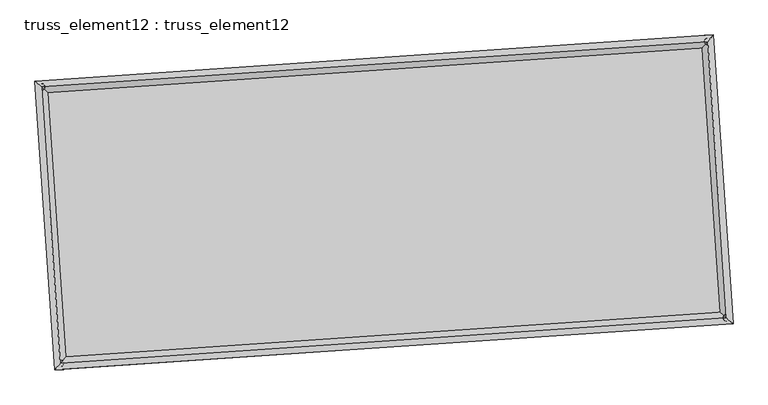
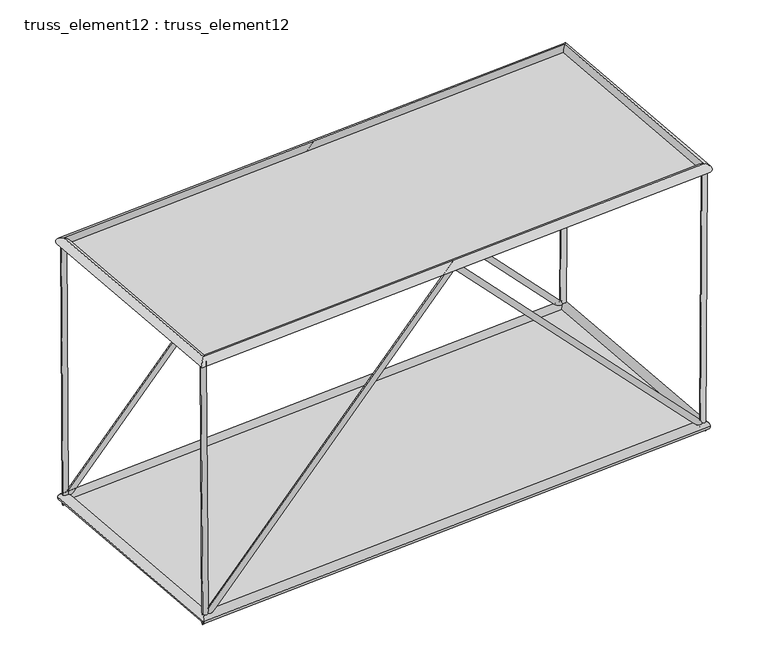
"""IFC4 building model written with IfcOpenShell, lengths in millimetres: plate geometry, truss_element12 : truss_element12."""

import ifcopenshell
import ifcopenshell.guid

model = None  # the IFC model being written
_history = None  # IfcOwnerHistory: only IFC2X3 demands one
_inside = {}  # id of a spatial element -> (the spatial element, [elements in it])
_under = {}  # id of a project, library or spatial element -> (it, [spatial elements below it])
_declared = {}  # id of a project -> (the project, [libraries it declares])
_typed = {}  # id of a type object -> (the type object, [elements of that type])
_made_of = {}  # id of a material, layer set ... -> (it, [elements and type objects made of it])


def new_model(schema):
    """Start an empty IFC model of exactly this schema.

    Asked for "IFC4X3", IfcOpenShell would pick the latest addendum, in which some entities
    have other attributes; the version numbers below select the first issue.
    IFC2X3 requires an IfcOwnerHistory on every rooted entity: one is made here for all.
    """
    global model, _history
    if schema == "IFC4X3":
        model = ifcopenshell.file(schema_version=(4, 3, 0, 0))
    else:
        model = ifcopenshell.file(schema=schema)
    _inside.clear()
    _under.clear()
    _declared.clear()
    _typed.clear()
    _made_of.clear()
    _history = None
    if model.schema == "IFC2X3":
        org = make("IfcOrganization", Name="unknown")
        user = make(
            "IfcPersonAndOrganization",
            ThePerson=make("IfcPerson", FamilyName="unknown"),
            TheOrganization=org,
        )
        app = make(
            "IfcApplication",
            ApplicationDeveloper=org,
            Version="unknown",
            ApplicationFullName="unknown",
            ApplicationIdentifier="unknown",
        )
        _history = make(
            "IfcOwnerHistory",
            OwningUser=user,
            OwningApplication=app,
            ChangeAction="ADDED",
            CreationDate=0,
        )
    return model


def make(cls, **values):
    """One entity of the class cls with the attributes given. An attribute that is None is left unset."""
    return model.create_entity(
        cls, **{name: value for name, value in values.items() if value is not None}
    )


def rooted(cls, **values):
    """An entity with a GlobalId (a new one), such as an element, a storey or a relation."""
    return make(cls, GlobalId=ifcopenshell.guid.new(), OwnerHistory=_history, **values)


def si_unit(unit_type, name, prefix=None):
    """IfcSIUnit, for example si_unit("LENGTHUNIT", "METRE", prefix="MILLI")."""
    return make("IfcSIUnit", UnitType=unit_type, Prefix=prefix, Name=name)


def assignment(units):
    """IfcUnitAssignment: the units of a project."""
    return None if units is None else make("IfcUnitAssignment", Units=units)


def point(xyz):
    """IfcCartesianPoint."""
    return None if xyz is None else make("IfcCartesianPoint", Coordinates=xyz)


def direction(xyz):
    """IfcDirection."""
    return None if xyz is None else make("IfcDirection", DirectionRatios=xyz)


def frame(location, z_axis=None, x_axis=None):
    """IfcAxis2Placement3D, a coordinate frame: its origin and axes. An axis left out is left unset."""
    return make(
        "IfcAxis2Placement3D",
        Location=point(location),
        Axis=direction(z_axis),
        RefDirection=direction(x_axis),
    )


def origin():
    """The frame at (0, 0, 0) with its axes left unset."""
    return frame((0.0, 0.0, 0.0))


def origin_with_axes():
    """The frame at (0, 0, 0) with the z axis (0, 0, 1) and the x axis (1, 0, 0) written out."""
    return frame((0.0, 0.0, 0.0), z_axis=(0.0, 0.0, 1.0), x_axis=(1.0, 0.0, 0.0))


def place(relative_to, where):
    """IfcLocalPlacement: puts the frame where relative to a parent placement (None: the world)."""
    return make(
        "IfcLocalPlacement", PlacementRelTo=relative_to, RelativePlacement=where
    )


def context(
    kind, dimensions, precision=None, world=None, true_north=None, identifier=None
):
    """IfcGeometricRepresentationContext, for example the 3D "Model" context."""
    return make(
        "IfcGeometricRepresentationContext",
        ContextIdentifier=identifier,
        ContextType=kind,
        CoordinateSpaceDimension=dimensions,
        Precision=precision,
        WorldCoordinateSystem=world,
        TrueNorth=true_north,
    )


def project(units=None, contexts=None):
    """IfcProject with its units and contexts."""
    return rooted(
        "IfcProject",
        Name="project",
        RepresentationContexts=contexts,
        UnitsInContext=assignment(units),
    )


def spatial(cls, under=None, at=None, **own):
    """A site, building, storey or space (cls), placed at a placement, below another one or the project."""
    s = rooted(cls, ObjectPlacement=at, **own)
    if under is not None:
        _under.setdefault(under.id(), (under, []))[1].append(s)
    return s


def polyline(points):
    """IfcPolyline through the points."""
    return make("IfcPolyline", Points=[point(p) for p in points])


def circle_curve(where, radius):
    """IfcCircle in the frame where."""
    return make("IfcCircle", Position=where, Radius=radius)


def ellipse_curve(where, semi_axis1, semi_axis2):
    """IfcEllipse in the frame where."""
    return make(
        "IfcEllipse", Position=where, SemiAxis1=semi_axis1, SemiAxis2=semi_axis2
    )


def outline(outer, holes=None, kind="AREA"):
    """IfcArbitraryClosedProfileDef: a profile drawn as a closed curve; with holes, ...WithVoids."""
    if holes is None:
        return make("IfcArbitraryClosedProfileDef", ProfileType=kind, OuterCurve=outer)
    return make(
        "IfcArbitraryProfileDefWithVoids",
        ProfileType=kind,
        OuterCurve=outer,
        InnerCurves=holes,
    )


def extrude(swept, where, along, depth):
    """IfcExtrudedAreaSolid: the profile swept, set in the frame where, extruded along a direction by depth."""
    return make(
        "IfcExtrudedAreaSolid",
        SweptArea=swept,
        Position=where,
        ExtrudedDirection=direction(along),
        Depth=depth,
    )


def shape(context_of_items, identifier, shape_type, items):
    """IfcShapeRepresentation: the items that make up one representation, for example the "Body"."""
    return make(
        "IfcShapeRepresentation",
        ContextOfItems=context_of_items,
        RepresentationIdentifier=identifier,
        RepresentationType=shape_type,
        Items=items,
    )


def source(mapping_origin, context_of_items, identifier, shape_type, items):
    """IfcRepresentationMap: a shape defined once, which mapped items show again and again."""
    return make(
        "IfcRepresentationMap",
        MappingOrigin=mapping_origin,
        MappedRepresentation=shape(context_of_items, identifier, shape_type, items),
    )


def transform(
    local_origin,
    x_axis=None,
    y_axis=None,
    z_axis=None,
    scale=None,
    scale2=None,
    scale3=None,
    uniform=True,
):
    """IfcCartesianTransformationOperator3D, or its non-uniform kind. x_axis, y_axis, z_axis: its Axis1, 2, 3."""
    if uniform:
        return make(
            "IfcCartesianTransformationOperator3D",
            Axis1=direction(x_axis),
            Axis2=direction(y_axis),
            LocalOrigin=point(local_origin),
            Scale=scale,
            Axis3=direction(z_axis),
        )
    return make(
        "IfcCartesianTransformationOperator3DnonUniform",
        Axis1=direction(x_axis),
        Axis2=direction(y_axis),
        LocalOrigin=point(local_origin),
        Scale=scale,
        Axis3=direction(z_axis),
        Scale2=scale2,
        Scale3=scale3,
    )


def mapped(mapping_source, mapping_target):
    """IfcMappedItem: shows the shape of a source again, moved by a transform."""
    return make(
        "IfcMappedItem", MappingSource=mapping_source, MappingTarget=mapping_target
    )


def made_of(thing, what):
    """Note that an element or type object is made of a material, layer set ...; save() writes the relation."""
    if what is not None:
        _made_of.setdefault(what.id(), (what, []))[1].append(thing)
    return thing


def element(
    cls,
    number,
    at=None,
    inside=None,
    cuts=None,
    type_object=None,
    material=None,
    context=None,
    identifier="Body",
    shape_type=None,
    held_by="IfcProductDefinitionShape",
    body=None,
    shapes=None,
    **own,
):
    """One element of the class cls, such as IfcWall. Its Tag is "e" and its number.

    at: its placement. inside: the storey or other place that contains it. cuts: it is an
    opening in that element (IfcRelVoidsElement). A single representation is given by context,
    identifier, shape_type and body (its items); several are given by shapes. held_by: the class
    of the entity that holds the representations. save() writes the other relations.
    """
    e = rooted(cls, Tag="e%d" % number, ObjectPlacement=at, **own)
    if body is not None:
        shapes = [shape(context, identifier, shape_type, body)]
    if shapes is not None:
        e.Representation = make(held_by, Representations=shapes)
    if inside is not None:
        _inside.setdefault(inside.id(), (inside, []))[1].append(e)
    if cuts is not None:
        rooted(
            "IfcRelVoidsElement", RelatingBuildingElement=cuts, RelatedOpeningElement=e
        )
    if type_object is not None:
        _typed.setdefault(type_object.id(), (type_object, []))[1].append(e)
    return made_of(e, material)


def aggregate(whole, parts):
    """IfcRelAggregates: a whole, such as a stair, and the parts it consists of."""
    return rooted("IfcRelAggregates", RelatingObject=whole, RelatedObjects=parts)


def save(model, path):
    """Write the relations noted so far, then the file.

    IfcRelAggregates (storeys below a building ...), IfcRelContainedInSpatialStructure (elements
    in a storey), IfcRelDefinesByType, IfcRelAssociatesMaterial and IfcRelDeclares: one each for
    every whole, place, type object, material and project.
    """
    for whole, parts in _under.values():
        aggregate(whole, parts)
    for where, things in _inside.values():
        rooted(
            "IfcRelContainedInSpatialStructure",
            RelatedElements=things,
            RelatingStructure=where,
        )
    for kind, things in _typed.values():
        rooted("IfcRelDefinesByType", RelatedObjects=things, RelatingType=kind)
    for what, things in _made_of.values():
        rooted("IfcRelAssociatesMaterial", RelatedObjects=things, RelatingMaterial=what)
    for by, libraries in _declared.values():
        rooted("IfcRelDeclares", RelatingContext=by, RelatedDefinitions=libraries)
    model.write(path)


def plane_surface(at):
    """IfcPlane: the flat surface through the origin of the frame at, square to its z axis."""
    return make("IfcPlane", Position=at)


def cylinder_surface(at, radius):
    """IfcCylindricalSurface: all points at the distance radius from the z axis of the frame at."""
    return make("IfcCylindricalSurface", Position=at, Radius=radius)


def advanced_brep(points, edges, surfaces, faces):
    """IfcAdvancedBrep: a solid bounded by faces that lie on surfaces and meet in shared edges.

    An edge is (start, end): straight between two places in points (the first is 0);
    or (start, end, curve); or (start, end, curve, False) where it runs against its curve.
    A face is (place in surfaces, loops), or (place, loops, False) where it looks against
    its surface's normal. A loop lists edges by number (the first is 1), with a minus sign
    where the edge is run from its end to its start. The first loop is the outer one.
    """
    corners = [point(p) for p in points]
    vertices = [make("IfcVertexPoint", VertexGeometry=c) for c in corners]
    made = []
    for start, end, *more in edges:
        made.append(
            make(
                "IfcEdgeCurve",
                EdgeStart=vertices[start],
                EdgeEnd=vertices[end],
                EdgeGeometry=more[0] if more else make("IfcPolyline", Points=[corners[start], corners[end]]),
                SameSense=more[1] if len(more) > 1 else True,
            )
        )
    hull = []
    for where, loops, *sense in faces:
        bounds = []
        for j, loop in enumerate(loops):
            ring = [make("IfcOrientedEdge", EdgeElement=made[abs(k) - 1], Orientation=k > 0) for k in loop]
            bounds.append(
                make(
                    "IfcFaceOuterBound" if j == 0 else "IfcFaceBound",
                    Bound=make("IfcEdgeLoop", EdgeList=ring),
                    Orientation=True,
                )
            )
        hull.append(make("IfcAdvancedFace", Bounds=bounds, FaceSurface=surfaces[where], SameSense=sense[0] if sense else True))
    return make("IfcAdvancedBrep", Outer=make("IfcClosedShell", CfsFaces=hull))


def truss_element12_truss_element12_7878418a(model_context):
    return source(origin(), model_context, "Body", "SolidModel", [
        advanced_brep(
        [(-3697.7330559, 2273.9880634, 5000.2199286), (-3796.8342671, 2260.6269358, 4999.5640296), (-3665.7497354, 2276.1688844, 123.3649597), (-3763.2371475, 2262.9177957, -123.3649597), (1063.4710215, 2598.6364704, 5072.016746), (1063.9229343, 2592.0634919, 4927.7704366), (5793.1764667, 2921.1371054, 123.3684641), (5891.5845103, 2921.2433831, -123.3684641), (5824.6787759, 2923.2851281, 5000.2182213), (5924.6764587, 2923.4997973, 4999.5721856)],
        [
            (0, 1, circle_curve(frame((-3747.2836615, 2267.3074996, 4999.8919791), z_axis=(-0.0065580440171227215, -0.0004471680920716447, 0.9999783958163132), x_axis=(-0.13361132201156306, 0.9910337164155191, -0.0004330796311214912)), 50.0)),
            (1, 0, circle_curve(frame((-3747.2836615, 2267.3074996, 4999.8919791), z_axis=(-0.0065580440171227215, -0.0004471680920716447, 0.9999783958163132), x_axis=(-0.13361132201156306, 0.9910337164155191, -0.0004330796311214912)), 50.0)),
            (0, 2),
            (2, 3, ellipse_curve(frame((-3714.4934414, 2269.54334, 0.0), z_axis=(-0.9270094873495339, -0.06320925304940259, 0.36967282925972605), x_axis=(0.36881644373245154, 0.025148191295556746, 0.9291619876572165)), 133.0592395, 50.0)),
            (3, 1),
            (3, 2, ellipse_curve(frame((-3714.4934414, 2269.54334, 0.0), z_axis=(-0.9270094873495339, -0.06320925304940259, 0.36967282925972605), x_axis=(0.36881644373245154, 0.025148191295556746, 0.9291619876572165)), 133.0592395, 50.0)),
            (2, 4),
            (4, 5, ellipse_curve(frame((1063.6969779, 2595.3499811, 4999.8935913), z_axis=(-0.9976833957434984, -0.06802823820610858, -2.5773915168840048e-05), x_axis=(2.571420721554706e-05, 1.7533540442212808e-06, -0.9999999996678525)), 72.2802032, 50.0)),
            (5, 3),
            (5, 4, ellipse_curve(frame((1063.6969779, 2595.3499811, 4999.8935913), z_axis=(-0.9976833957434984, -0.06802823820610858, -2.5773915168840048e-05), x_axis=(2.571420721554706e-05, 1.7533540442212808e-06, -0.9999999996678525)), 72.2802032, 50.0)),
            (4, 6),
            (6, 7, ellipse_curve(frame((5842.3804885, 2921.1902443, 0.0), z_axis=(-0.9269817502517963, -0.06320736176214367, -0.3697426998862667), x_axis=(-0.36888615249642426, -0.025152944471190097, 0.929134186154408)), 133.0670008, 50.0)),
            (7, 5),
            (7, 6, ellipse_curve(frame((5842.3804885, 2921.1902443, 0.0), z_axis=(-0.9269817502517963, -0.06320736176214367, -0.3697426998862667), x_axis=(-0.36888615249642426, -0.025152944471190097, 0.929134186154408)), 133.0670008, 50.0)),
            (8, 9, circle_curve(frame((5874.6776173, 2923.3924627, 4999.8952035), z_axis=(0.0064594257599789005, 0.0004404436879936221, 0.9999790406944584), x_axis=(-0.002149492172002672, 0.9999975988590792, -0.00042656708586943926)), 50.0)),
            (9, 8, circle_curve(frame((5874.6776173, 2923.3924627, 4999.8952035), z_axis=(0.0064594257599789005, 0.0004404436879936221, 0.9999790406944584), x_axis=(-0.002149492172002672, 0.9999975988590792, -0.00042656708586943926)), 50.0)),
            (6, 8),
            (9, 7),
        ],
        [
            plane_surface(frame((-3747.2836615, 2317.3074946, 4999.914338), z_axis=(-0.006558044017122149, -0.0004471680920756006, 0.9999783958163133), x_axis=(0.9999784957981195, -2.932611094408344e-06, 0.0065580433614229605))),
            cylinder_surface(frame((-3747.2836615, 2267.3074996, 4999.8919791), z_axis=(-0.0065580440171227215, -0.0004471680920716447, 0.9999783958163132), x_axis=(-0.13361132201156306, 0.9910337164155191, -0.0004330796311214912)), 50.0),
            cylinder_surface(frame((-3714.4934414, 2269.54334, 0.0), z_axis=(-0.6901312584427534, -0.047057427078693426, -0.722152646382297), x_axis=(-0.02041166390988012, 0.9987523707892875, -0.045574837566446924)), 50.0),
            cylinder_surface(frame((1063.6969779, 2595.3499811, 4999.8935913), z_axis=(-0.6901683966914209, -0.047059959394698786, 0.7221169880498334), x_axis=(-0.11534684875831876, 0.9922791014168952, -0.04557729009939607)), 50.0),
            plane_surface(frame((5874.6776173, 2873.3924675, 4999.9172261), z_axis=(0.006459425759978055, 0.0004404436879920798, 0.9999790406944582), x_axis=(0.9999791376918077, -2.845072659241059e-06, -0.006459425133417806))),
            cylinder_surface(frame((5842.3804885, 2921.1902443, 0.0), z_axis=(-0.0064594257599789005, -0.0004404436879936221, -0.9999790406944584), x_axis=(-0.002149492172002672, 0.9999975988590792, -0.00042656708586943926)), 50.0),
        ],
        [
            (0, [[1, 2]]),
            (1, [[-1, 3, 4, 5]]),
            (1, [[-2, -5, 6, -3]]),
            (2, [[-4, 7, 8, 9]]),
            (2, [[-6, -9, 10, -7]]),
            (3, [[-8, 11, 12, 13]]),
            (3, [[-10, -13, 14, -11]]),
            (4, [[15, 16]]),
            (5, [[-12, 17, -16, 18]]),
            (5, [[-14, -18, -15, -17]]),
        ],
    ),
        advanced_brep(
        [(-3425.620103, -1716.7455209, 5000.2199286), (-3524.7213142, -1730.1066485, 4999.5640296), (-3393.6367824, -1714.5646999, 123.3649597), (-3491.1241946, -1727.8157886, -123.3649597), (1335.5839744, -1392.0971139, 5072.016746), (1336.0358872, -1398.6700924, 4927.7704366), (6065.2894196, -1069.5964789, 123.3684641), (6163.6974632, -1069.4902012, -123.3684641), (6096.7917288, -1067.4484562, 5000.2182213), (6196.7894116, -1067.233787, 4999.5721856)],
        [
            (0, 1, circle_curve(frame((-3475.1707086, -1723.4260847, 4999.8919791), z_axis=(-0.006558044017122952, -0.00044716809207167603, 0.9999783958163132), x_axis=(-0.1336113220115621, 0.9910337164155192, -0.0004330796311214846)), 50.0)),
            (1, 0, circle_curve(frame((-3475.1707086, -1723.4260847, 4999.8919791), z_axis=(-0.006558044017122952, -0.00044716809207167603, 0.9999783958163132), x_axis=(-0.1336113220115621, 0.9910337164155192, -0.0004330796311214846)), 50.0)),
            (0, 2),
            (2, 3, ellipse_curve(frame((-3442.3804885, -1721.1902443, 0.0), z_axis=(-0.927009487349534, -0.06320925304940223, 0.3696728292597261), x_axis=(0.3688164437324516, 0.025148191295556586, 0.9291619876572165)), 133.0592395, 50.0)),
            (3, 1),
            (3, 2, ellipse_curve(frame((-3442.3804885, -1721.1902443, 0.0), z_axis=(-0.927009487349534, -0.06320925304940223, 0.3696728292597261), x_axis=(0.3688164437324516, 0.025148191295556586, 0.9291619876572165)), 133.0592395, 50.0)),
            (2, 4),
            (4, 5, ellipse_curve(frame((1335.8099308, -1395.3836032, 4999.8935913), z_axis=(-0.9976833957434985, -0.06802823820610843, -2.5773915170605434e-05), x_axis=(2.5714207217238277e-05, 1.7533540445864214e-06, -0.9999999996678526)), 72.2802032, 50.0)),
            (5, 3),
            (5, 4, ellipse_curve(frame((1335.8099308, -1395.3836032, 4999.8935913), z_axis=(-0.9976833957434985, -0.06802823820610843, -2.5773915170605434e-05), x_axis=(2.5714207217238277e-05, 1.7533540445864214e-06, -0.9999999996678526)), 72.2802032, 50.0)),
            (4, 6),
            (6, 7, ellipse_curve(frame((6114.4934414, -1069.54334, 0.0), z_axis=(-0.9269817502517956, -0.06320736176214367, -0.3697426998862684), x_axis=(-0.3688861524964258, -0.025152944471190226, 0.9291341861544073)), 133.0670008, 50.0)),
            (7, 5),
            (7, 6, ellipse_curve(frame((6114.4934414, -1069.54334, 0.0), z_axis=(-0.9269817502517956, -0.06320736176214367, -0.3697426998862684), x_axis=(-0.3688861524964258, -0.025152944471190226, 0.9291341861544073)), 133.0670008, 50.0)),
            (8, 9, circle_curve(frame((6146.7905702, -1067.3411216, 4999.8952035), z_axis=(0.006459425759979071, 0.0004404436879936256, 0.9999790406944583), x_axis=(-0.002149492172003178, 0.9999975988590791, -0.00042656708586943915)), 50.0)),
            (9, 8, circle_curve(frame((6146.7905702, -1067.3411216, 4999.8952035), z_axis=(0.006459425759979071, 0.0004404436879936256, 0.9999790406944583), x_axis=(-0.002149492172003178, 0.9999975988590791, -0.00042656708586943915)), 50.0)),
            (6, 8),
            (9, 7),
        ],
        [
            plane_surface(frame((-3475.1707086, -1673.4260897, 4999.914338), z_axis=(-0.006558044017122149, -0.00044716809207560177, 0.9999783958163133), x_axis=(0.9999784957981195, -2.932611094408344e-06, 0.0065580433614229605))),
            cylinder_surface(frame((-3475.1707086, -1723.4260847, 4999.8919791), z_axis=(-0.0065580440171229505, -0.0004471680920716759, 0.999978395816313), x_axis=(-0.1336113220115621, 0.9910337164155192, -0.0004330796311214846)), 50.0),
            cylinder_surface(frame((-3442.3804885, -1721.1902443, 0.0), z_axis=(-0.6901312584427537, -0.04705742707869316, -0.7221526463822968), x_axis=(-0.020411663909880064, 0.9987523707892874, -0.045574837566446605)), 50.0),
            cylinder_surface(frame((1335.8099308, -1395.3836032, 4999.8935913), z_axis=(-0.6901683966914235, -0.047059959394698994, 0.7221169880498306), x_axis=(-0.1153468487583182, 0.9922791014168953, -0.045577290099395824)), 50.0),
            plane_surface(frame((6146.7905702, -1117.3411168, 4999.9172261), z_axis=(0.006459425759978055, 0.00044044368799207986, 0.9999790406944582), x_axis=(0.9999791376918077, -2.8450726587969697e-06, -0.006459425133417806))),
            cylinder_surface(frame((6114.4934414, -1069.54334, 0.0), z_axis=(-0.006459425759979071, -0.0004404436879936256, -0.9999790406944583), x_axis=(-0.002149492172003178, 0.9999975988590791, -0.00042656708586943915)), 50.0),
        ],
        [
            (0, [[1, 2]]),
            (1, [[-1, 3, 4, 5]]),
            (1, [[-2, -5, 6, -3]]),
            (2, [[-4, 7, 8, 9]]),
            (2, [[-6, -9, 10, -7]]),
            (3, [[-8, 11, 12, 13]]),
            (3, [[-10, -13, 14, -11]]),
            (4, [[15, 16]]),
            (5, [[-12, 17, -16, 18]]),
            (5, [[-14, -18, -15, -17]]),
        ],
    ),
        advanced_brep(
        [(-3475.1698571, -1723.425141, 4909.8919791), (-3475.1715601, -1723.4270284, 5089.8919791), (-3747.2846332, 2267.308319, 5089.8919791), (-3747.2826898, 2267.3066802, 4909.8919791), (5874.6784087, 2923.3934023, 5089.8952035), (5874.6768259, 2923.3915231, 4909.8952035), (6146.7914819, -1067.3419451, 5089.8952035), (6146.7896586, -1067.3402981, 4909.8952035)],
        [
            (0, 1, ellipse_curve(frame((-3475.1707086, -1723.4260847, 4999.8919791), z_axis=(-0.7535719234054182, 0.6573654662780838, -2.364078017319096e-07), x_axis=(-0.6573654662780416, -0.7535719234054551, -2.3640780134907803e-07)), 127.2792206, 90.0)),
            (1, 2),
            (2, 3, ellipse_curve(frame((-3747.2836615, 2267.3074996, 4999.8919791), z_axis=(-0.6573654662780415, -0.7535719234054551, -2.3640779880847992e-07), x_axis=(0.7535719234054182, -0.6573654662780839, 2.3640779919131162e-07)), 127.2792206, 90.0)),
            (3, 0),
            (1, 0, ellipse_curve(frame((-3475.1707086, -1723.4260847, 4999.8919791), z_axis=(-0.7535719234054182, 0.6573654662780838, -2.364078017319096e-07), x_axis=(-0.6573654662780416, -0.7535719234054551, -2.3640780134907803e-07)), 127.2792206, 90.0)),
            (3, 2, ellipse_curve(frame((-3747.2836615, 2267.3074996, 4999.8919791), z_axis=(-0.6573654662780415, -0.7535719234054551, -2.3640779880847992e-07), x_axis=(0.7535719234054182, -0.6573654662780839, 2.3640779919131162e-07)), 127.2792206, 90.0)),
            (2, 4),
            (4, 5, ellipse_curve(frame((5874.6776173, 2923.3924627, 4999.8952035), z_axis=(-0.753571923405421, 0.6573654662780805, -2.364078053169509e-07), x_axis=(-0.6573654662780386, -0.7535719234054576, -2.3640779268284074e-07)), 127.2792206, 90.0)),
            (5, 3),
            (5, 4, ellipse_curve(frame((5874.6776173, 2923.3924627, 4999.8952035), z_axis=(-0.753571923405421, 0.6573654662780805, -2.364078053169509e-07), x_axis=(-0.6573654662780386, -0.7535719234054576, -2.3640779268284074e-07)), 127.2792206, 90.0)),
            (4, 6),
            (6, 7, ellipse_curve(frame((6146.7905702, -1067.3411216, 4999.8952035), z_axis=(0.6573654662780387, 0.7535719234054576, 2.3640779522343875e-07), x_axis=(-0.7535719234054211, 0.6573654662780807, -2.364078078575489e-07)), 127.2792206, 90.0)),
            (7, 5),
            (7, 6, ellipse_curve(frame((6146.7905702, -1067.3411216, 4999.8952035), z_axis=(0.6573654662780387, 0.7535719234054576, 2.3640779522343875e-07), x_axis=(-0.7535719234054211, 0.6573654662780807, -2.364078078575489e-07)), 127.2792206, 90.0)),
            (6, 1),
            (0, 7),
        ],
        [
            cylinder_surface(frame((-3475.1707086, -1723.4260847, 4999.8919791), z_axis=(0.06802823822870056, -0.9976833960748767, 0.0), x_axis=(-0.9976833960234631, -0.06802823822519488, -1.0152132427543063e-05)), 90.0),
            cylinder_surface(frame((-3747.2836615, 2267.3074996, 4999.8919791), z_axis=(-0.9976833960748208, -0.06802823822869773, -3.3433111559642525e-07), x_axis=(-0.06802823822214815, 0.9976833960270169, -9.817801312233482e-06)), 90.0),
            cylinder_surface(frame((5874.6776173, 2923.3924627, 4999.8952035), z_axis=(-0.06802823822870865, 0.9976833960748761, 0.0), x_axis=(0.9976833960300122, 0.06802823822564956, -9.48347018771953e-06)), 90.0),
            cylinder_surface(frame((6146.7905702, -1067.3411216, 4999.8952035), z_axis=(0.997683396074821, 0.06802823822869727, 3.3433111918937347e-07), x_axis=(0.06802823822869727, -0.9976833960265705, -9.81780129795915e-06)), 90.0),
        ],
        [
            (0, [[1, 2, 3, 4]]),
            (0, [[5, -4, 6, -2]]),
            (1, [[-3, 7, 8, 9]]),
            (1, [[-6, -9, 10, -7]]),
            (2, [[-8, 11, 12, 13]]),
            (2, [[-10, -13, 14, -11]]),
            (3, [[-12, 15, -1, 16]]),
            (3, [[-14, -16, -5, -15]]),
        ],
    ),
        advanced_brep(
        [(-3358.7115243, -1625.2761972, 0.0), (-3526.0494527, -1817.1042913, 0.0), (-3810.4074885, 2353.2123043, 0.0), (-3618.5793943, 2185.8743758, 0.0), (5926.0494527, 3017.1042913, 0.0), (5758.7115243, 2825.2761972, 0.0), (6210.4074885, -1153.2123043, 0.0), (6018.5793943, -985.8743758, 0.0)],
        [
            (0, 1, ellipse_curve(frame((-3442.3804885, -1721.1902443, 0.0), z_axis=(-0.7535719234054593, 0.6573654662780792, 0.0), x_axis=(-0.6573654662780792, -0.7535719234054593, 0.0)), 127.2792206, 90.0)),
            (1, 2),
            (2, 3, ellipse_curve(frame((-3714.4934414, 2269.54334, 0.0), z_axis=(-0.6573654662780791, -0.7535719234054593, 0.0), x_axis=(0.7535719234054593, -0.6573654662780793, 0.0)), 127.2792206, 90.0)),
            (3, 0),
            (1, 0, ellipse_curve(frame((-3442.3804885, -1721.1902443, 0.0), z_axis=(-0.7535719234054593, 0.6573654662780792, 0.0), x_axis=(-0.6573654662780792, -0.7535719234054593, 0.0)), 127.2792206, 90.0)),
            (3, 2, ellipse_curve(frame((-3714.4934414, 2269.54334, 0.0), z_axis=(-0.6573654662780791, -0.7535719234054593, 0.0), x_axis=(0.7535719234054593, -0.6573654662780793, 0.0)), 127.2792206, 90.0)),
            (2, 4),
            (4, 5, ellipse_curve(frame((5842.3804885, 2921.1902443, 0.0), z_axis=(-0.7535719234054621, 0.6573654662780759, 0.0), x_axis=(-0.6573654662780762, -0.753571923405462, 0.0)), 127.2792206, 90.0)),
            (5, 3),
            (5, 4, ellipse_curve(frame((5842.3804885, 2921.1902443, 0.0), z_axis=(-0.7535719234054621, 0.6573654662780759, 0.0), x_axis=(-0.6573654662780762, -0.753571923405462, 0.0)), 127.2792206, 90.0)),
            (4, 6),
            (6, 7, ellipse_curve(frame((6114.4934414, -1069.54334, 0.0), z_axis=(0.6573654662780762, 0.7535719234054619, 0.0), x_axis=(-0.753571923405462, 0.6573654662780763, 0.0)), 127.2792206, 90.0)),
            (7, 5),
            (7, 6, ellipse_curve(frame((6114.4934414, -1069.54334, 0.0), z_axis=(0.6573654662780762, 0.7535719234054619, 0.0), x_axis=(-0.753571923405462, 0.6573654662780763, 0.0)), 127.2792206, 90.0)),
            (6, 1),
            (0, 7),
        ],
        [
            cylinder_surface(frame((-3442.3804885, -1721.1902443, 0.0), z_axis=(0.06802823822870308, -0.9976833960748764, 0.0), x_axis=(-0.9976833960748764, -0.06802823822870308, 0.0)), 90.0),
            cylinder_surface(frame((-3714.4934414, 2269.54334, 0.0), z_axis=(-0.9976833960748765, -0.06802823822870399, 0.0), x_axis=(-0.06802823822870399, 0.9976833960748765, 0.0)), 90.0),
            cylinder_surface(frame((5842.3804885, 2921.1902443, 0.0), z_axis=(-0.06802823822871121, 0.997683396074876, 0.0), x_axis=(0.997683396074876, 0.06802823822871121, 0.0)), 90.0),
            cylinder_surface(frame((6114.4934414, -1069.54334, 0.0), z_axis=(0.9976833960748765, 0.06802823822870341, 0.0), x_axis=(0.06802823822870341, -0.9976833960748765, 0.0)), 90.0),
        ],
        [
            (0, [[1, 2, 3, 4]]),
            (0, [[5, -4, 6, -2]]),
            (1, [[-3, 7, 8, 9]]),
            (1, [[-6, -9, 10, -7]]),
            (2, [[-8, 11, 12, 13]]),
            (2, [[-10, -13, 14, -11]]),
            (3, [[-12, 15, -1, 16]]),
            (3, [[-14, -16, -5, -15]]),
        ],
    ),
        extrude(outline(polyline([(-3442.3804885, -1721.1902443), (-3714.4934414, 2269.54334), (5842.3804885, 2921.1902443), (6114.4934414, -1069.54334), (-3442.3804885, -1721.1902443)])), origin_with_axes(), (0.0, 0.0, 1.0), 20.0),
        extrude(outline(polyline([(-2000.0, 4822.1516549), (2000.0, 4822.1516549), (2000.0, -4822.1516548), (-2000.0, -4822.1516548), (-2000.0, 4822.1516549)])), frame((1199.7534544, 599.983189, 4999.8935913), z_axis=(-3.33556602840147e-07, -2.2743956508971097e-08, 0.9999999999999442), x_axis=(-0.06802823822870292, 0.9976833960748765, 0.0)), (0.0, 0.0, 1.0), 20.0),
    ])


if __name__ == "__main__":
    model = new_model("IFC4")
    model_context = context("Model", 3, world=origin())
    ifc_project = project(units=[si_unit("LENGTHUNIT", "METRE", prefix="MILLI")], contexts=[model_context])
    site = spatial("IfcSite", under=ifc_project)
    building = spatial("IfcBuilding", under=site)
    placement = place(None, origin())
    truss_element12_truss_element12_shape = truss_element12_truss_element12_7878418a(model_context)
    element("IfcPlate", 1, ObjectType="truss_element12 : truss_element12", at=placement, inside=building, context=model_context, shape_type="MappedRepresentation", body=[
        mapped(truss_element12_truss_element12_shape, transform((0.0, 0.0, 0.0), x_axis=(1.0, 0.0, 0.0), y_axis=(0.0, 1.0, 0.0), z_axis=(0.0, 0.0, 1.0))),
    ])
    save(model, "model.ifc")

# Revit data of these elements
# Type "truss_element12 : truss_element12"
#   steellbar1 = 90 mm
#   steelbar2 = 50 mm
#   offset1 = 5000 mm
#   M = Default Roof
# Element 1 (IfcPlate, "truss_element12 : truss_element12")
#   Materials on its faces: "Default Roof"
# Materials
#   "Default Roof": class "Miscellaneous", colour RGB 0 127 0, transparency 0, Comments = "Rendering appearance not upgraded Rendering appearance not upgraded ", Cost = 0
